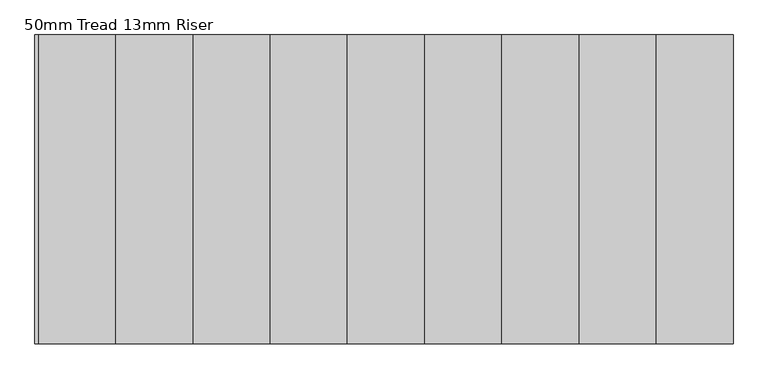
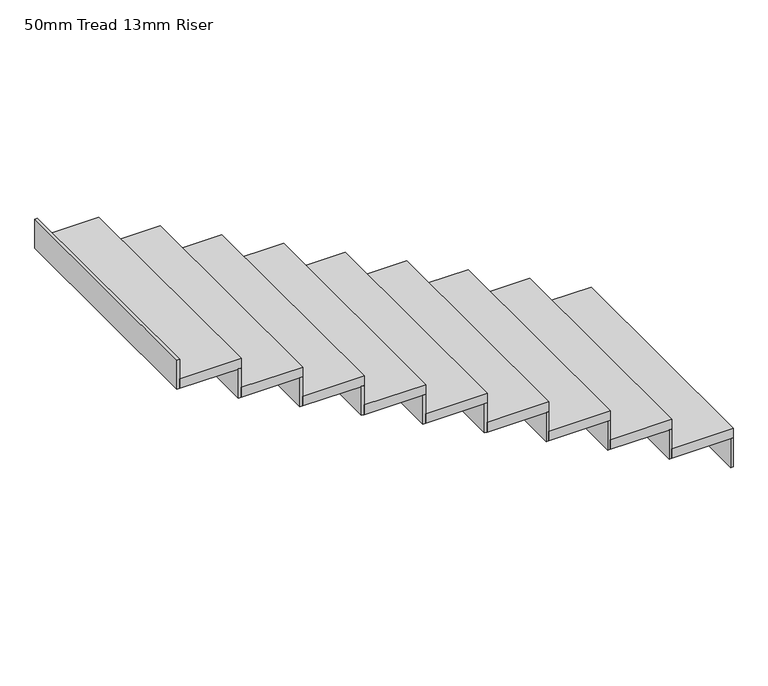
"""IFC4 building model written with IfcOpenShell, lengths in millimetres: stair flight geometry, 50mm Tread 13mm Riser."""

from ifc_helpers import new_model, si_unit, frame, origin, place, context, project, spatial, polyline, outline, extrude, source, transform, mapped, element, save


def stair_flight_50mm_tread_13mm_riser_c3aae4ce(model_context):
    return source(origin(), model_context, "Body", "SweptSolid", [
        extrude(outline(polyline([(18583.7289955, -4912.5395691), (18596.2289955, -4912.5395691), (18596.2289955, -6112.5395691), (18583.7289955, -6112.5395691), (18583.7289955, -4912.5395691)])), frame((0.0, 0.0, 1450.0), z_axis=(0.0, 0.0, 1.0), x_axis=(1.0, 0.0, 0.0)), (0.0, 0.0, 1.0), 150.0),
        extrude(outline(polyline([(18296.2289955, -6112.5395691), (18296.2289955, -4912.5395691), (18596.2289955, -4912.5395691), (18596.2289955, -6112.5395691), (18296.2289955, -6112.5395691)])), frame((0.0, 0.0, 1600.0), z_axis=(0.0, 0.0, 1.0), x_axis=(1.0, 0.0, 0.0)), (0.0, 0.0, 1.0), 50.0),
        extrude(outline(polyline([(18283.7289955, -4912.5395691), (18296.2289955, -4912.5395691), (18296.2289955, -6112.5395691), (18283.7289955, -6112.5395691), (18283.7289955, -4912.5395691)])), frame((0.0, 0.0, 1600.0), z_axis=(0.0, 0.0, 1.0), x_axis=(1.0, 0.0, 0.0)), (0.0, 0.0, 1.0), 150.0),
        extrude(outline(polyline([(17996.2289955, -6112.5395691), (17996.2289955, -4912.5395691), (18296.2289955, -4912.5395691), (18296.2289955, -6112.5395691), (17996.2289955, -6112.5395691)])), frame((0.0, 0.0, 1750.0), z_axis=(0.0, 0.0, 1.0), x_axis=(1.0, 0.0, 0.0)), (0.0, 0.0, 1.0), 50.0),
        extrude(outline(polyline([(17983.7289955, -4912.5395691), (17996.2289955, -4912.5395691), (17996.2289955, -6112.5395691), (17983.7289955, -6112.5395691), (17983.7289955, -4912.5395691)])), frame((0.0, 0.0, 1750.0), z_axis=(0.0, 0.0, 1.0), x_axis=(1.0, 0.0, 0.0)), (0.0, 0.0, 1.0), 150.0),
        extrude(outline(polyline([(17696.2289955, -6112.5395691), (17696.2289955, -4912.5395691), (17996.2289955, -4912.5395691), (17996.2289955, -6112.5395691), (17696.2289955, -6112.5395691)])), frame((0.0, 0.0, 1900.0), z_axis=(0.0, 0.0, 1.0), x_axis=(1.0, 0.0, 0.0)), (0.0, 0.0, 1.0), 50.0),
        extrude(outline(polyline([(17683.7289955, -4912.5395691), (17696.2289955, -4912.5395691), (17696.2289955, -6112.5395691), (17683.7289955, -6112.5395691), (17683.7289955, -4912.5395691)])), frame((0.0, 0.0, 1900.0), z_axis=(0.0, 0.0, 1.0), x_axis=(1.0, 0.0, 0.0)), (0.0, 0.0, 1.0), 150.0),
        extrude(outline(polyline([(17396.2289955, -6112.5395691), (17396.2289955, -4912.5395691), (17696.2289955, -4912.5395691), (17696.2289955, -6112.5395691), (17396.2289955, -6112.5395691)])), frame((0.0, 0.0, 2050.0), z_axis=(0.0, 0.0, 1.0), x_axis=(1.0, 0.0, 0.0)), (0.0, 0.0, 1.0), 50.0),
        extrude(outline(polyline([(17383.7289955, -4912.5395691), (17396.2289955, -4912.5395691), (17396.2289955, -6112.5395691), (17383.7289955, -6112.5395691), (17383.7289955, -4912.5395691)])), frame((0.0, 0.0, 2050.0), z_axis=(0.0, 0.0, 1.0), x_axis=(1.0, 0.0, 0.0)), (0.0, 0.0, 1.0), 150.0),
        extrude(outline(polyline([(17096.2289955, -6112.5395691), (17096.2289955, -4912.5395691), (17396.2289955, -4912.5395691), (17396.2289955, -6112.5395691), (17096.2289955, -6112.5395691)])), frame((0.0, 0.0, 2200.0), z_axis=(0.0, 0.0, 1.0), x_axis=(1.0, 0.0, 0.0)), (0.0, 0.0, 1.0), 50.0),
        extrude(outline(polyline([(17083.7289955, -4912.5395691), (17096.2289955, -4912.5395691), (17096.2289955, -6112.5395691), (17083.7289955, -6112.5395691), (17083.7289955, -4912.5395691)])), frame((0.0, 0.0, 2200.0), z_axis=(0.0, 0.0, 1.0), x_axis=(1.0, 0.0, 0.0)), (0.0, 0.0, 1.0), 150.0),
        extrude(outline(polyline([(16796.2289955, -6112.5395691), (16796.2289955, -4912.5395691), (17096.2289955, -4912.5395691), (17096.2289955, -6112.5395691), (16796.2289955, -6112.5395691)])), frame((0.0, 0.0, 2350.0), z_axis=(0.0, 0.0, 1.0), x_axis=(1.0, 0.0, 0.0)), (0.0, 0.0, 1.0), 50.0),
        extrude(outline(polyline([(16783.7289955, -4912.5395691), (16796.2289955, -4912.5395691), (16796.2289955, -6112.5395691), (16783.7289955, -6112.5395691), (16783.7289955, -4912.5395691)])), frame((0.0, 0.0, 2350.0), z_axis=(0.0, 0.0, 1.0), x_axis=(1.0, 0.0, 0.0)), (0.0, 0.0, 1.0), 150.0),
        extrude(outline(polyline([(16496.2289955, -6112.5395691), (16496.2289955, -4912.5395691), (16796.2289955, -4912.5395691), (16796.2289955, -6112.5395691), (16496.2289955, -6112.5395691)])), frame((0.0, 0.0, 2500.0), z_axis=(0.0, 0.0, 1.0), x_axis=(1.0, 0.0, 0.0)), (0.0, 0.0, 1.0), 50.0),
        extrude(outline(polyline([(16483.7289955, -4912.5395691), (16496.2289955, -4912.5395691), (16496.2289955, -6112.5395691), (16483.7289955, -6112.5395691), (16483.7289955, -4912.5395691)])), frame((0.0, 0.0, 2500.0), z_axis=(0.0, 0.0, 1.0), x_axis=(1.0, 0.0, 0.0)), (0.0, 0.0, 1.0), 150.0),
        extrude(outline(polyline([(16196.2289955, -6112.5395691), (16196.2289955, -4912.5395691), (16496.2289955, -4912.5395691), (16496.2289955, -6112.5395691), (16196.2289955, -6112.5395691)])), frame((0.0, 0.0, 2650.0), z_axis=(0.0, 0.0, 1.0), x_axis=(1.0, 0.0, 0.0)), (0.0, 0.0, 1.0), 50.0),
        extrude(outline(polyline([(16183.7289955, -4912.5395691), (16196.2289955, -4912.5395691), (16196.2289955, -6112.5395691), (16183.7289955, -6112.5395691), (16183.7289955, -4912.5395691)])), frame((0.0, 0.0, 2650.0), z_axis=(0.0, 0.0, 1.0), x_axis=(1.0, 0.0, 0.0)), (0.0, 0.0, 1.0), 150.0),
        extrude(outline(polyline([(15883.7289955, -4912.5395691), (15896.2289955, -4912.5395691), (15896.2289955, -6112.5395691), (15883.7289955, -6112.5395691), (15883.7289955, -4912.5395691)])), frame((0.0, 0.0, 2800.0), z_axis=(0.0, 0.0, 1.0), x_axis=(1.0, 0.0, 0.0)), (0.0, 0.0, 1.0), 150.0),
        extrude(outline(polyline([(15896.2289955, -6112.5395691), (15896.2289955, -4912.5395691), (16196.2289955, -4912.5395691), (16196.2289955, -6112.5395691), (15896.2289955, -6112.5395691)])), frame((0.0, 0.0, 2800.0), z_axis=(0.0, 0.0, 1.0), x_axis=(1.0, 0.0, 0.0)), (0.0, 0.0, 1.0), 50.0),
    ])


if __name__ == "__main__":
    model = new_model("IFC4")
    model_context = context("Model", 3, world=origin())
    ifc_project = project(units=[si_unit("LENGTHUNIT", "METRE", prefix="MILLI")], contexts=[model_context])
    site = spatial("IfcSite", under=ifc_project)
    building = spatial("IfcBuilding", under=site)
    placement = place(None, origin())
    stair_flight_50mm_tread_13mm_riser_shape = stair_flight_50mm_tread_13mm_riser_c3aae4ce(model_context)
    element("IfcStairFlight", 1, ObjectType="50mm Tread 13mm Riser", at=placement, inside=building, context=model_context, shape_type="MappedRepresentation", body=[
        mapped(stair_flight_50mm_tread_13mm_riser_shape, transform((0.0, 0.0, 0.0), x_axis=(1.0, 0.0, 0.0), y_axis=(0.0, 1.0, 0.0), z_axis=(0.0, 0.0, 1.0))),
    ])
    save(model, "model.ifc")
